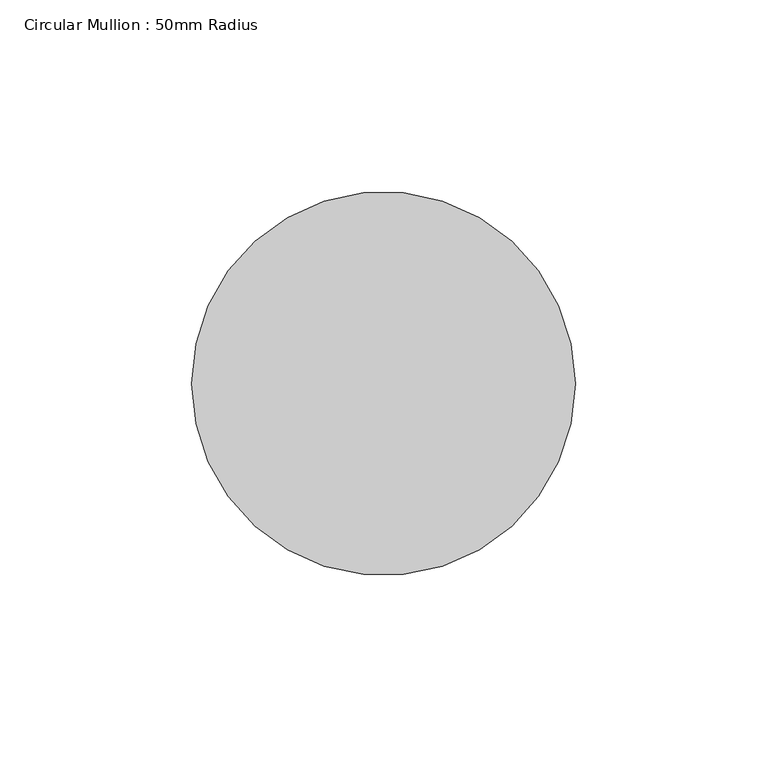
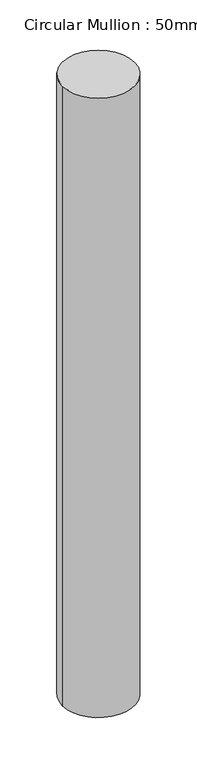
"""IFC4 building model written with IfcOpenShell, lengths in millimetres: member geometry, Circular Mullion : 50mm Radius."""

from ifc_helpers import new_model, si_unit, point, frame, origin, origin_2d, place, context, project, spatial, circle_curve, trimmed, segment, composite_curve, outline, extrude, source, transform, mapped, element, save


def circular_mullion_50mm_radius_c331aff3(model_context):
    return source(origin(), model_context, "Body", "SweptSolid", [
        extrude(outline(composite_curve([segment(trimmed(circle_curve(origin_2d(), 50.0), [point((50.0, 0.0))], [point((-50.0, 0.0))], False, "CARTESIAN"), True, "CONTINUOUS"), segment(trimmed(circle_curve(origin_2d(), 50.0), [point((-50.0, 0.0))], [point((50.0, 0.0))], False, "CARTESIAN"), True, "CONTINUOUS")], self_intersect=False)), frame((0.0, 0.0, -908.9766943), z_axis=(0.0, 0.0, 1.0), x_axis=(1.0, 0.0, 0.0)), (0.0, 0.0, 1.0), 908.9766943),
    ])


if __name__ == "__main__":
    model = new_model("IFC4")
    model_context = context("Model", 3, world=origin())
    ifc_project = project(units=[si_unit("LENGTHUNIT", "METRE", prefix="MILLI")], contexts=[model_context])
    site = spatial("IfcSite", under=ifc_project)
    building = spatial("IfcBuilding", under=site)
    placement = place(None, origin())
    circular_mullion_50mm_radius_shape = circular_mullion_50mm_radius_c331aff3(model_context)
    element("IfcMember", 1, ObjectType="Circular Mullion : 50mm Radius", at=placement, inside=building, context=model_context, shape_type="MappedRepresentation", body=[
        mapped(circular_mullion_50mm_radius_shape, transform((0.0, 0.0, 0.0), x_axis=(1.0, 0.0, 0.0), y_axis=(0.0, 1.0, 0.0), z_axis=(0.0, 0.0, 1.0))),
    ])
    save(model, "model.ifc")

# Revit data of these elements
# Type "Circular Mullion : 50mm Radius"
#   built-in parameter 1007350 = 0.164042 (stored number, unit not read)
# Element 1 (IfcMember, "Circular Mullion : 50mm Radius")
#   Materials on its faces: "Aluminium"
# Materials
#   "Aluminium": class "Metal", colour RGB 247 247 247, transparency 0, Description = "Aluminium 6061", Cost = 0
